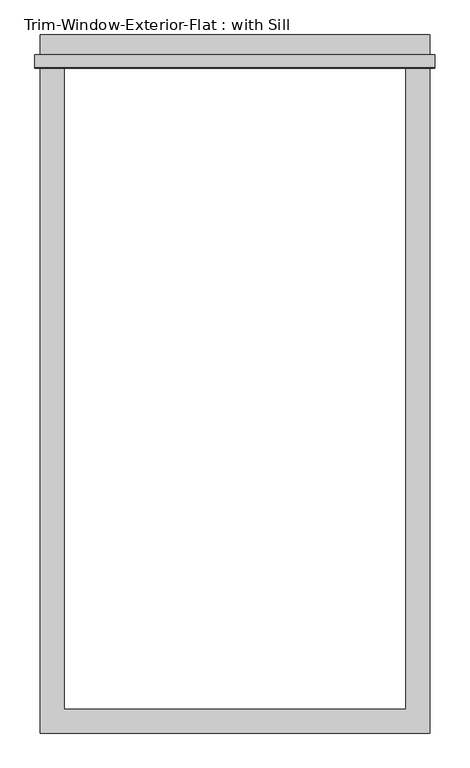
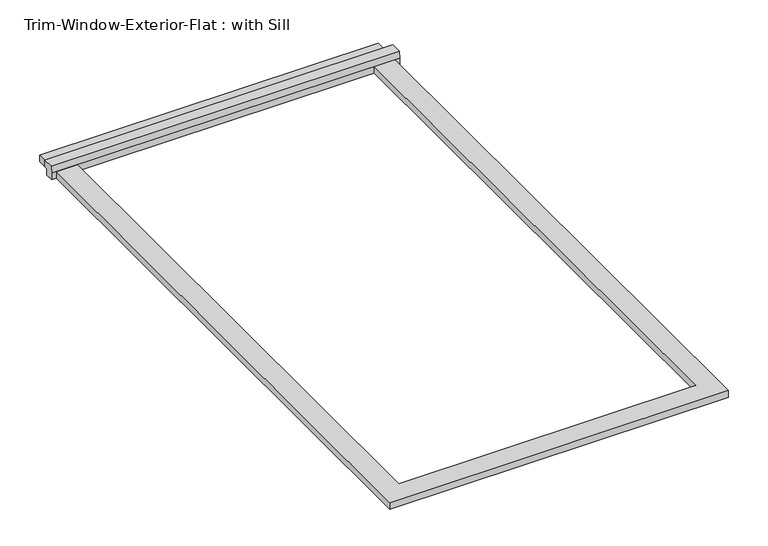
"""IFC4 building model written with IfcOpenShell, lengths in millimetres: proxy geometry, Trim-Window-Exterior-Flat : with Sill."""

from ifc_helpers import new_model, si_unit, frame, origin, origin_with_axes, place, context, project, spatial, polyline, outline, extrude, source, transform, mapped, element, save


def trim_window_exterior_flat_with_sill_16e6dc7d(model_context):
    return source(origin(), model_context, "Body", "SweptSolid", [
        extrude(outline(polyline([(463.55, 1546.1823709), (-463.55, 1546.1823709), (-463.55, 1603.3323709), (463.55, 1603.3323709), (463.55, 1546.1823709)])), origin_with_axes(), (0.0, 0.0, 1.0), 19.05),
        extrude(outline(polyline([(1555.75, 38.1), (1555.75, 19.05), (1546.1823709, 19.05), (1546.1823709, 0.0), (1524.0, 0.0), (1524.0, 19.05), (1526.4580645, 38.1), (1555.75, 38.1)])), frame((-476.25, 0.0, 0.0), z_axis=(1.0, 0.0, 0.0), x_axis=(0.0, 1.0, 0.0)), (0.0, 0.0, 1.0), 952.5),
        extrude(outline(polyline([(-463.55, -57.15), (-463.55, 1524.0), (-406.4, 1524.0), (-406.4, 0.0), (406.4, 0.0), (406.4, 1524.0), (463.55, 1524.0), (463.55, -57.15), (-463.55, -57.15)])), origin_with_axes(), (0.0, 0.0, 1.0), 19.05),
    ])


if __name__ == "__main__":
    model = new_model("IFC4")
    model_context = context("Model", 3, world=origin())
    ifc_project = project(units=[si_unit("LENGTHUNIT", "METRE", prefix="MILLI")], contexts=[model_context])
    site = spatial("IfcSite", under=ifc_project)
    building = spatial("IfcBuilding", under=site)
    placement = place(None, origin())
    trim_window_exterior_flat_with_sill_shape = trim_window_exterior_flat_with_sill_16e6dc7d(model_context)
    element("IfcBuildingElementProxy", 1, Name="Trim-Window-Exterior-Flat : with Sill", ObjectType="Trim-Window-Exterior-Flat : with Sill", at=placement, inside=building, context=model_context, shape_type="MappedRepresentation", body=[
        mapped(trim_window_exterior_flat_with_sill_shape, transform((0.0, 0.0, 0.0), x_axis=(1.0, 0.0, 0.0), y_axis=(0.0, 1.0, 0.0), z_axis=(0.0, 0.0, 1.0))),
    ])
    save(model, "model.ifc")

# Revit data of these elements
# Type "Trim-Window-Exterior-Flat : with Sill"
#   Trim Width = 0' - 2 1/4"
#   Trim Thickness_Picture Frame = 0' - 1 1/4"
#   Trim Thickness_with Sill = 0' - 0 3/4"
#   Sill Thickness = 0' - 1 1/4"
#   Opening Width [instance default] = 2' - 0"
#   Opening Height [instance default] = 3' - 0"
#   Default Elevation = 4' - 0"
#   Sill = yes
#   Picture Frame = no
#   Trim Material [instance default] = none
# Element 1 (IfcBuildingElementProxy, "Trim-Window-Exterior-Flat : with Sill")
#   Opening Width = 2' - 8"
#   Opening Height = 5' - 0"
#   Trim Material = Clad - White
#   Materials on its faces: "Clad - White"
# Materials
#   "Clad - White": class "Wood", colour RGB 242 242 238, transparency 0, Cost = 0
